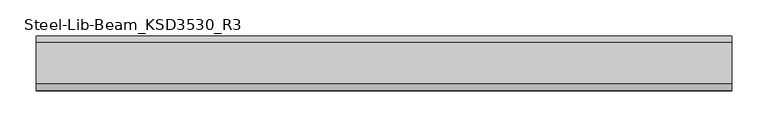
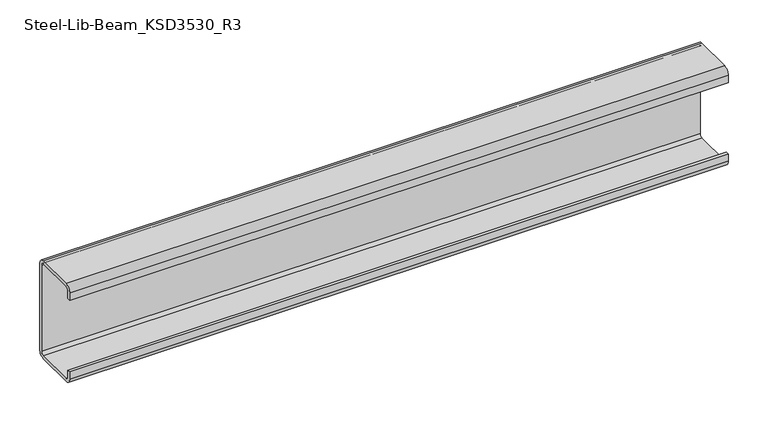
"""IFC4 building model written with IfcOpenShell, lengths in millimetres: beam geometry, Steel-Lib-Beam_KSD3530_R3 : BMS291_C-150×75x20x4.5."""

from ifc_helpers import new_model, si_unit, point, frame, frame_2d, origin, place, context, project, spatial, polyline, circle_curve, trimmed, segment, composite_curve, outline, extrude, source, transform, mapped, element, save


def steel_lib_beam_ksd3530_r3_86accbbc(model_context):
    return source(origin(), model_context, "Body", "SweptSolid", [
        extrude(outline(composite_curve([segment(trimmed(circle_curve(frame_2d((-41.0, 66.0)), 9.0), [point((-50.0, 66.0))], [point((-41.0, 75.0))], False, "CARTESIAN"), True, "CONTINUOUS"), segment(polyline([(-41.0, 75.0), (16.0, 75.0)]), True, "CONTINUOUS"), segment(trimmed(circle_curve(frame_2d((16.0, 66.0)), 9.0), [point((16.0, 75.0))], [point((25.0, 66.0))], False, "CARTESIAN"), True, "CONTINUOUS"), segment(polyline([(25.0, 66.0), (25.0, -66.0)]), True, "CONTINUOUS"), segment(trimmed(circle_curve(frame_2d((16.0, -66.0)), 9.0), [point((25.0, -66.0))], [point((16.0, -75.0))], False, "CARTESIAN"), True, "CONTINUOUS"), segment(polyline([(16.0, -75.0), (-41.0, -75.0)]), True, "CONTINUOUS"), segment(trimmed(circle_curve(frame_2d((-41.0, -66.0)), 9.0), [point((-41.0, -75.0))], [point((-50.0, -66.0))], False, "CARTESIAN"), True, "CONTINUOUS"), segment(polyline([(-50.0, -66.0), (-50.0, -55.0), (-45.5, -55.0), (-45.5, -66.0)]), True, "CONTINUOUS"), segment(trimmed(circle_curve(frame_2d((-41.0, -66.0)), 4.5), [point((-45.5, -66.0))], [point((-41.0, -70.5))], True, "CARTESIAN"), True, "CONTINUOUS"), segment(polyline([(-41.0, -70.5), (16.0, -70.5)]), True, "CONTINUOUS"), segment(trimmed(circle_curve(frame_2d((16.0, -66.0)), 4.5), [point((16.0, -70.5))], [point((20.5, -66.0))], True, "CARTESIAN"), True, "CONTINUOUS"), segment(polyline([(20.5, -66.0), (20.5, 66.0)]), True, "CONTINUOUS"), segment(trimmed(circle_curve(frame_2d((16.0, 66.0)), 4.5), [point((20.5, 66.0))], [point((16.0, 70.5))], True, "CARTESIAN"), True, "CONTINUOUS"), segment(polyline([(16.0, 70.5), (-41.0, 70.5)]), True, "CONTINUOUS"), segment(trimmed(circle_curve(frame_2d((-41.0, 66.0)), 4.5), [point((-41.0, 70.5))], [point((-45.5, 66.0))], True, "CARTESIAN"), True, "CONTINUOUS"), segment(polyline([(-45.5, 66.0), (-45.5, 55.0), (-50.0, 55.0), (-50.0, 66.0)]), True, "CONTINUOUS")], self_intersect=False)), frame((-477.5, 0.0, 0.0), z_axis=(1.0, 0.0, 0.0), x_axis=(0.0, 1.0, 0.0)), (0.0, 0.0, 1.0), 955.0),
    ])


if __name__ == "__main__":
    model = new_model("IFC4")
    model_context = context("Model", 3, world=origin())
    ifc_project = project(units=[si_unit("LENGTHUNIT", "METRE", prefix="MILLI")], contexts=[model_context])
    site = spatial("IfcSite", under=ifc_project)
    building = spatial("IfcBuilding", under=site)
    placement = place(None, origin())
    steel_lib_beam_ksd3530_r3_shape = steel_lib_beam_ksd3530_r3_86accbbc(model_context)
    element("IfcBeam", 1, ObjectType="Steel-Lib-Beam_KSD3530_R3 : BMS291_C-150×75x20x4.5", at=placement, inside=building, context=model_context, shape_type="MappedRepresentation", body=[
        mapped(steel_lib_beam_ksd3530_r3_shape, transform((0.0, 0.0, 0.0), x_axis=(1.0, 0.0, 0.0), y_axis=(0.0, 1.0, 0.0), z_axis=(0.0, 0.0, 1.0))),
    ])
    save(model, "model.ifc")

# Revit data of these elements
# Type "Steel-Lib-Beam_KSD3530_R3 : BMS291_C-150×75x20x4.5"
#   Keynote = "C-150×75x20x4.5"
#   SteelWeight = "Light"
#   x = 0.0250 m
#   t1 = 0.0090 m
#   t = 0.0045 m
#   Surface Area = 0.629834 m²/m
#   Section Area = 13.9688 cm²
#   Mass per Unit Length = 10.9655 kg/m
#   C = 0.0200 m
#   A = 0.0750 m
#   Length [instance default] = 1.5000 m
#   H = 0.1500 m
#   hec_material4 [instance default] = none
#   hec_material3 [instance default] = none
#   hec_material2 [instance default] = none
#   hec_material1 [instance default] = none
#   Structural Material [instance default] = Metal - Steel - Light Gauge
#   Assembly Code = ""
# Element 1 (IfcBeam, "Steel-Lib-Beam_KSD3530_R3 : BMS291_C-150×75x20x4.5")
#   Structural Material = none
# Materials
#   "Metal - Steel - Light Gauge": class "Metal", colour RGB 247 247 247, transparency 0
